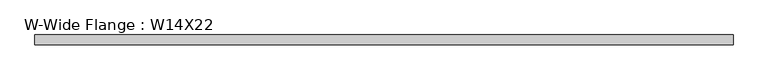
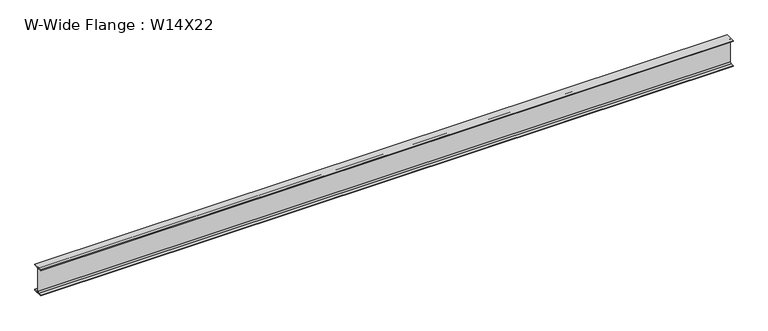
"""IFC4 building model written with IfcOpenShell, lengths in millimetres: beam geometry, W-Wide Flange : W14X22."""

from ifc_helpers import new_model, si_unit, point, frame, frame_2d, origin, place, context, project, spatial, polyline, circle_curve, trimmed, segment, composite_curve, outline, extrude, source, transform, mapped, element, save


def w_wide_flange_w14x22_ec72dc32(model_context):
    return source(origin(), model_context, "Body", "SweptSolid", [
        extrude(outline(composite_curve([segment(polyline([(63.5, -165.481), (63.5, -173.99), (-63.5, -173.99), (-63.5, -165.481), (-21.3995, -165.481)]), True, "CONTINUOUS"), segment(trimmed(circle_curve(frame_2d((-21.3995, -147.0025)), 18.4785), [point((-21.3995, -165.481))], [point((-2.921, -147.0025))], True, "CARTESIAN"), True, "CONTINUOUS"), segment(polyline([(-2.921, -147.0025), (-2.921, 147.0025)]), True, "CONTINUOUS"), segment(trimmed(circle_curve(frame_2d((-21.3995, 147.0025)), 18.4785), [point((-2.921, 147.0025))], [point((-21.3995, 165.481))], True, "CARTESIAN"), True, "CONTINUOUS"), segment(polyline([(-21.3995, 165.481), (-63.5, 165.481), (-63.5, 173.99), (63.5, 173.99), (63.5, 165.481), (21.3995, 165.481)]), True, "CONTINUOUS"), segment(trimmed(circle_curve(frame_2d((21.3995, 147.0025)), 18.4785), [point((21.3995, 165.481))], [point((2.921, 147.0025))], True, "CARTESIAN"), True, "CONTINUOUS"), segment(polyline([(2.921, 147.0025), (2.921, -147.0025)]), True, "CONTINUOUS"), segment(trimmed(circle_curve(frame_2d((21.3995, -147.0025)), 18.4785), [point((2.921, -147.0025))], [point((21.3995, -165.481))], True, "CARTESIAN"), True, "CONTINUOUS"), segment(polyline([(21.3995, -165.481), (63.5, -165.481)]), True, "CONTINUOUS")], self_intersect=False)), frame((-4406.646, 0.0, 0.0), z_axis=(1.0, 0.0, 0.0), x_axis=(0.0, 1.0, 0.0)), (0.0, 0.0, 1.0), 8813.292),
    ])


if __name__ == "__main__":
    model = new_model("IFC4")
    model_context = context("Model", 3, world=origin())
    ifc_project = project(units=[si_unit("LENGTHUNIT", "METRE", prefix="MILLI")], contexts=[model_context])
    site = spatial("IfcSite", under=ifc_project)
    building = spatial("IfcBuilding", under=site)
    placement = place(None, origin())
    w_wide_flange_w14x22_shape = w_wide_flange_w14x22_ec72dc32(model_context)
    element("IfcBeam", 1, ObjectType="W-Wide Flange : W14X22", at=placement, inside=building, context=model_context, shape_type="MappedRepresentation", body=[
        mapped(w_wide_flange_w14x22_shape, transform((0.0, 0.0, 0.0), x_axis=(1.0, 0.0, 0.0), y_axis=(0.0, 1.0, 0.0), z_axis=(0.0, 0.0, 1.0))),
    ])
    save(model, "model.ifc")

# Revit data of these elements
# Type "W-Wide Flange : W14X22"
#   Assembly Code = "B10"
#   W = 22
#   Length [instance default] = 1524 mm
#   bf = 127 mm
#   d = 347.98 mm
#   k = 26.988 mm
#   k2 = 18.479 mm
#   tf = 8.509 mm
#   tw = 5.842 mm
#   A = 0.00418709 m²
#   Structural Material [instance default] = Steel ASTM A992
# Element 1 (IfcBeam, "W-Wide Flange : W14X22")
#   Structural Material = Aluminum, Anodized Red
#   Materials on its faces: "Aluminum, Anodized Red"
# Materials
#   "Steel ASTM A992": class "Metal", colour RGB 128 0 0, transparency 0, Description = "Structural steel 50ksi", Cost = 0
#   "Aluminum, Anodized Red": class "Metal", colour RGB 120 120 120, transparency 0, Description = "Anodized aluminum, red", Cost = 0
